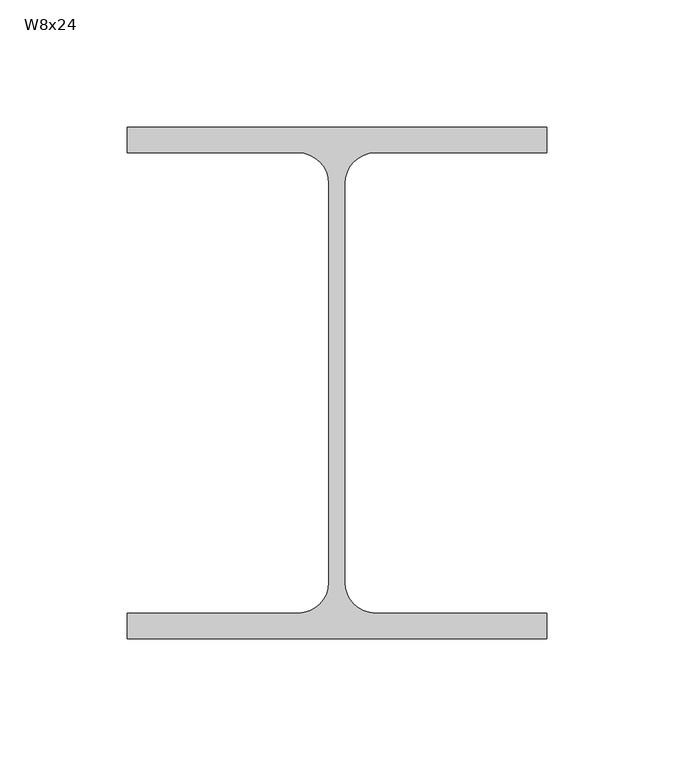
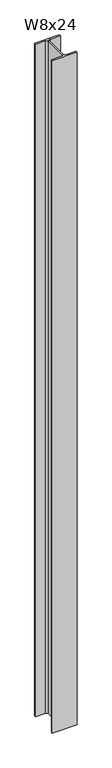
"""IFC4 building model written with IfcOpenShell, lengths in millimetres: column geometry, RME WF - Column : W8x24."""

from ifc_helpers import new_model, si_unit, point, frame, frame_2d, origin, place, context, project, spatial, polyline, circle_curve, trimmed, segment, composite_curve, outline, extrude, source, transform, mapped, element, save


def w8x24_7aa3e7e1(model_context):
    return source(origin(), model_context, "Body", "SweptSolid", [
        extrude(outline(composite_curve([segment(polyline([(82.55, 100.711), (82.55, 90.551), (15.1765, 90.551)]), True, "CONTINUOUS"), segment(trimmed(circle_curve(frame_2d((15.1765, 78.486)), 12.065), [point((15.1765, 90.551))], [point((3.1115, 78.486))], True, "CARTESIAN"), True, "CONTINUOUS"), segment(polyline([(3.1115, 78.486), (3.1115, -78.486)]), True, "CONTINUOUS"), segment(trimmed(circle_curve(frame_2d((15.1765, -78.486)), 12.065), [point((3.1115, -78.486))], [point((15.1765, -90.551))], True, "CARTESIAN"), True, "CONTINUOUS"), segment(polyline([(15.1765, -90.551), (82.55, -90.551), (82.55, -100.711), (-82.55, -100.711), (-82.55, -90.551), (-15.1765, -90.551)]), True, "CONTINUOUS"), segment(trimmed(circle_curve(frame_2d((-15.1765, -78.486)), 12.065), [point((-15.1765, -90.551))], [point((-3.1115, -78.486))], True, "CARTESIAN"), True, "CONTINUOUS"), segment(polyline([(-3.1115, -78.486), (-3.1115, 78.486)]), True, "CONTINUOUS"), segment(trimmed(circle_curve(frame_2d((-15.1765, 78.486)), 12.065), [point((-3.1115, 78.486))], [point((-15.1765, 90.551))], True, "CARTESIAN"), True, "CONTINUOUS"), segment(polyline([(-15.1765, 90.551), (-82.55, 90.551), (-82.55, 100.711), (82.55, 100.711)]), True, "CONTINUOUS")], self_intersect=False)), frame((0.0, 0.0, -304.8), z_axis=(0.0, 0.0, 1.0), x_axis=(1.0, 0.0, 0.0)), (0.0, 0.0, 1.0), 4718.05),
    ])


if __name__ == "__main__":
    model = new_model("IFC4")
    model_context = context("Model", 3, world=origin())
    ifc_project = project(units=[si_unit("LENGTHUNIT", "METRE", prefix="MILLI")], contexts=[model_context])
    site = spatial("IfcSite", under=ifc_project)
    building = spatial("IfcBuilding", under=site)
    placement = place(None, origin())
    w8x24_shape = w8x24_7aa3e7e1(model_context)
    element("IfcColumn", 1, ObjectType="RME WF - Column : W8x24", at=placement, inside=building, context=model_context, shape_type="MappedRepresentation", body=[
        mapped(w8x24_shape, transform((0.0, 0.0, 0.0), x_axis=(1.0, 0.0, 0.0), y_axis=(0.0, 1.0, 0.0), z_axis=(0.0, 0.0, 1.0))),
    ])
    save(model, "model.ifc")

# Revit data of these elements
# Type "RME WF - Column : W8x24"
#   Type Mark = "C1"
#   REINF TYPE [instance default] = ""
#   Nominal Size = "W16"
#   COL REMARKS [instance default] = ""
#   BP [instance default] = ""
#   Assembly Code = "B10"
#   W = 24
#   bf = 0' - 6 1/2"
#   d = 0' - 7.93"
#   k = 0' - 0 7/8"
#   kr = 0' - 0.475"
#   tf = 0' - 0.4"
#   tw = 0' - 0.245"
#   A = 0.0491667 SF
#   Structural Material [instance default] = Metal - Steel - ASTM A992
# Element 1 (IfcColumn, "RME WF - Column : W8x24")
#   Materials on its faces: "Metal - Steel - ASTM A992"
# Materials
#   "Metal - Steel - ASTM A992": class "Metal", colour RGB 255 128 0, transparency 0
